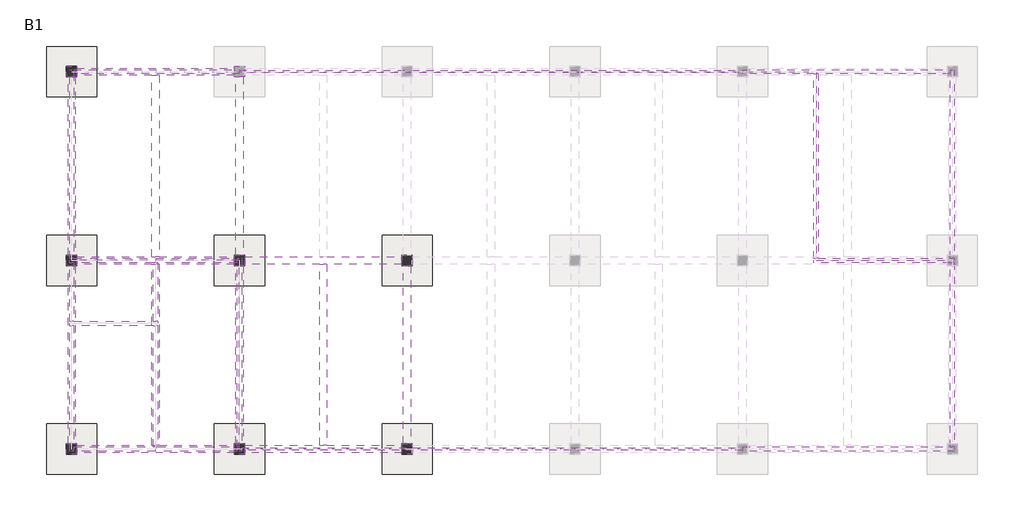
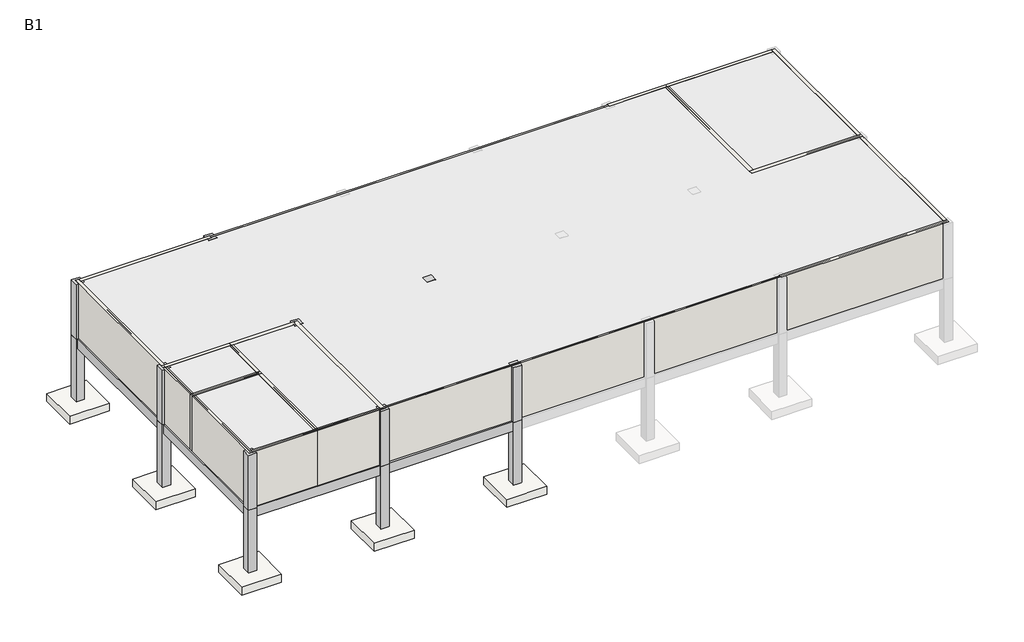
# One storey, part 1 of 2: 20 walls, 15 columns, 13 beams, 12 slabs.
# Revit data of these elements (continued)
# Elements 29, 30, 31, 32, 33 (IfcSlab, "CFS11_Slab RC_T150")
#   Height Offset From Level = 0 mm
#   Phase Created = New Construction
#   Materials on its faces: "14200-030101_Concrete Pouring"
# Elements 34, 35, 36, 37, 38, 39, 40 (IfcSlab, "FT112-Footing-Rectangular : FT112_2400x2400x500")
#   Comments = ""
#   hec_material3 = none
#   hec_material2 = none
#   hec_material1 = none
#   Structural Material = 콘크리트 - 현장타설 콘크리트
#   Phase Created = New Construction
#   Materials on its faces: "콘크리트 - 현장타설 콘크리트"
# Elements 41, 43, 46, 47, 49, 50 (IfcWall, "WA111-Exterior RC Wall 200mm")
#   Top Offset = 0 mm
#   Base Offset = 0 mm
#   Unconnected Height = 3500 mm
#   wall height = 3500 mm
#   Phase Created = New Construction
#   Base Constraint = GF
#   Materials on its faces: "Default Wall", "A03AD032-00007_Structural Concrete_25MPa-30MPa"
# Elements 42, 44, 45, 48 (IfcWall, "WA111-Exterior RC Wall 200mm")
#   Top Offset = 0 mm
#   Base Offset = 0 mm
#   Unconnected Height = 3500 mm
#   wall height = 3500 mm
#   Phase Created = New Construction
#   Base Constraint = GF
#   Materials on its faces: "A03AD032-00007_Structural Concrete_25MPa-30MPa", "Default Wall"
# Elements 51, 52 (IfcWall, "WA211_Exterior-Cement Brick-90mm")
#   Top Offset = 0 mm
#   Base Offset = 0 mm
#   Unconnected Height = 3500 mm
#   wall height = 3500 mm
#   Phase Created = New Construction
#   Base Constraint = GF
#   Materials on its faces: "Default Wall", "A04AS164-00002_Plastering_Int", "A04AS164-00001_Plastering_Ext"
# Elements 53, 56, 57, 58 (IfcWall, "WA221_Interior-Cement Block-190mm")
#   Top Offset = 0 mm
#   Base Offset = 0 mm
#   Unconnected Height = 3500 mm
#   wall height = 3500 mm
#   Phase Created = New Construction
#   Base Constraint = GF
#   Materials on its faces: "Default Wall", "A04AS164-00002_Plastering_Int"
# Elements 54, 55, 60 (IfcWall, "WA221_Interior-Cement Block-190mm")
#   Top Offset = 0 mm
#   Base Offset = 0 mm
#   Unconnected Height = 3500 mm
#   wall height = 3500 mm
#   Phase Created = New Construction
#   Base Constraint = GF
#   Materials on its faces: "A04AS164-00002_Plastering_Int", "Default Wall", "A03AD032-00007_Structural Concrete_25MPa-30MPa"
# Element 59 (IfcWall, "WA221_Interior-Cement Block-190mm")
#   Top Offset = 0 mm
#   Base Offset = 0 mm
#   Unconnected Height = 3500 mm
#   wall height = 3500 mm
#   Phase Created = New Construction
#   Base Constraint = GF
#   Materials on its faces: "Default Wall", "A04AS164-00002_Plastering_Int", "A03AD032-00007_Structural Concrete_25MPa-30MPa"
# Materials
#   "콘크리트 - 현장타설 콘크리트": class "콘크리트", colour RGB 192 192 192, transparency 0
#   "A03AE056-00001_Bitumen/Bituminous/Asphalt Coating": class "Generic", colour RGB 17 17 17, transparency 0, Description = "Damp-proofing", W00) Work Master Code = "A03AE056-00001", W01) Work Master_Lv1 = "Concrete Work", W02) Work Master_Lv2 = "Concrete Protective Coating (U/G)", W03) Work Master_Spec.1 = "Bitumen/Bituminous/Asphalt Coating", Cost = 0
#   "A03AC035-00001_Form Work (3 times in use)_Flat": class "Wood", colour RGB 149 120 74, transparency 0, Description = "Plywood", W00) Work Master Code = "A03AC035-00001", W01) Work Master_Lv1 = "Concrete Work", W02) Work Master_Lv2 = "Substructure Work", W03) Work Master_Spec.1 = "Form Work (3 times in use)", W04) Work Master_Spec.2 = "Flat Form", W05) Work Master_Spec.3 = "Dressed Lumber, Plywood or Steel Form(Wood Planks are not Allowed) incl. Chamfer", Cost = 0
#   "A03AC032-00007_Structural Concrete_Type1_25MPa-30Mpa": class "Concrete", colour RGB 176 176 176, transparency 0, Keynote = "09910.A1", Description = "Reinf. Conc.", W00) Work Master Code = "A03AC032-00007", W01) Work Master_Lv1 = "Concrete Work", W02) Work Master_Lv2 = "Substructure Work", W03) Work Master_Spec.1 = "Structural Concrete", W04) Work Master_Spec.2 = "Cement Type-1", W05) Work Master_Spec.3 = "25MPa < F'c (Cylinder Strength) ≤ 30MPa", Cost = 0
#   "14200-030101_Concrete Pouring": class "Concrete", colour RGB 176 176 176, transparency 0, Description = "Reinf. Conc.", W00) Work Master Code = "14200-030101", W01) Work Master_Lv1 = "Concrete Work", W02) Work Master_Lv2 = "Building/Shelter Foundation Work", W03) Work Master_Spec.1 = "Concrete Pouring", W04) Work Master_Spec.2 = "F'c (Cylinder Strength) > 35MPa", W05) Work Master_Spec.3 = "Cement Type-1", Cost = 0
#   "A04AL077-00001_Ext Wall Painting_Acrylic Emulsion Paint": class "Finish", colour RGB 128 128 64, transparency 0, Description = "Plastic", W00) Work Master Code = "A04AL077-00001", W01) Work Master_Lv1 = "Finishing Work", W02) Work Master_Lv2 = "Painting Work", W03) Work Master_Spec.1 = "External Wall Painting", W04) Work Master_Spec.2 = "Acrylic Emulsion Paint", Cost = 0
#   "A03AD032-00007_Structural Concrete_25MPa-30MPa": class "Concrete", colour RGB 176 176 176, transparency 0, Keynote = "09910.A1", Description = "LATEX PAINT ON F.F CONC.", W00) Work Master Code = "A03AD032-00007", W01) Work Master_Lv1 = "Concrete Work", W02) Work Master_Lv2 = "Superstructure Work", W03) Work Master_Spec.1 = "Structural Concrete", W04) Work Master_Spec.2 = "Cement Type-1", W05) Work Master_Spec.3 = "25MPa < F'c (Cylinder Strength) ≤ 30MPa", Cost = 0
#   "A03AD036-00001_Form Work (1 time in use)": class "Wood", colour RGB 149 120 74, transparency 0, Description = "Plywood", W00) Work Master Code = "A03AD036-00001", W01) Work Master_Lv1 = "Concrete Work", W02) Work Master_Lv2 = "Superstructure Work", W03) Work Master_Spec.1 = "Form Work (1 time in use)", W04) Work Master_Spec.2 = "Flat Form", W05) Work Master_Spec.3 = "Dressed Lumber, Plywood or Steel Form(Wood Planks are not Allowed) incl. Chamfer", Cost = 0
#   "A04AL078-00002_Int Wall Painting_Water Emulsion Paint": class "Finish", colour RGB 128 128 64, transparency 0, Description = "Plastic", W00) Work Master Code = "A04AL078-00002", W01) Work Master_Lv1 = "Finishing Work", W02) Work Master_Lv2 = "Painting Work", W03) Work Master_Spec.1 = "Internal Wall Painting", W04) Work Master_Spec.2 = "Water Emulsion Paint", Cost = 0
#   "A04AL081-00001_Skirt_Acrylic Emulsion Paint": class "Finish", colour RGB 128 128 64, transparency 0, Description = "Plastic", W00) Work Master Code = "A04AL081-00001", W01) Work Master_Lv1 = "Finishing Work", W02) Work Master_Lv2 = "Painting Work", W03) Work Master_Spec.1 = "Skirt Painting", W04) Work Master_Spec.2 = "Acrylic Emulsion Paint", W05) Work Master_Spec.3 = "100mm≤H<150mm", Cost = 0
#   "A04AS164-00001_Plastering_Ext": class "Concrete", colour RGB 183 186 184, transparency 0, W00) Work Master Code = "A04AS164-00001", W01) Work Master_Lv1 = "Finishing Work", W02) Work Master_Lv2 = "Plastering Work", W03) Work Master_Spec.1 = "Plastering", W04) Work Master_Spec.2 = "for External Masonry Wall", Cost = 0
#   "A04AK073-00001_Concrete Brick_0.5B": class "Concrete", colour RGB 180 180 180, transparency 0, Description = "Conc. Block", W00) Work Master Code = "A04AK073-00001", W01) Work Master_Lv1 = "Finishing Work", W02) Work Master_Lv2 = "Masonry Work", W03) Work Master_Spec.1 = "Concrete Brick", W04) Work Master_Spec.2 = "[0.5B] w/ All Reinf.(Lath, Steel Tie, Anchor Bar, Mortar, ETC.), Filler, Sealant, Lintel/Sill for Opening, ETC.", Cost = 0
#   "A04AS164-00002_Plastering_Int": class "Concrete", colour RGB 183 186 184, transparency 0, Description = "LATEX PAINT ON THK.15 CEMENT PLASTER", W00) Work Master Code = "A04AS164-00002", W01) Work Master_Lv1 = "Finishing Work", W02) Work Master_Lv2 = "Plastering Work", W03) Work Master_Spec.1 = "Plastering", W04) Work Master_Spec.2 = "for Internal Masonry Wall", Cost = 0
#   "A04AK069-00002_Reinforced Concrete Block_THK 100-200mm": class "Concrete", colour RGB 180 180 180, transparency 0, Description = "Conc. Block", W00) Work Master Code = "A04AK069-00002", W01) Work Master_Lv1 = "Finishing Work", W02) Work Master_Lv2 = "Masonry Work", W03) Work Master_Spec.1 = "Reinforced Concrete Block", W04) Work Master_Spec.2 = "w/ All Reinf.(Lath, Steel Tie, Anchor Bar, Mortar, ETC.), Filler, Sealant, Lintel/Sill for Opening, ETC.", W05) Work Master_Spec.3 = "100mm<THK≤200mm", Cost = 0
#   "Default Wall": class "Miscellaneous", colour RGB 80 80 80, transparency 0
# Room at (84209.652, 177423.861) mm, phase "New Construction", upper offset 3500 mm, lower offset 0 mm
#   Department = "EL"
#   Base Finish = ""
#   Ceiling Finish = "CL2"
#   Wall Finish = "IW2"
#   Floor Finish = "FL7"
#   Number = "0.0"
#   Name = "Battery Room"
#   Interior Finish = "IW2..N/A..N/A,,N/A..N/A,,FL7..N/A,,CL2..N/A"
#   Exterior Finish = "N/A..N/A,,EW2..N/A..N/A"
# Room at (51459.652, 168423.861) mm, phase "New Construction", upper offset 3500 mm, lower offset 0 mm
#   Department = "AR"
#   Base Finish = "WK3"
#   Ceiling Finish = ""
#   Wall Finish = "IW5"
#   Floor Finish = "FL2"
#   Number = "0.1"
#   Name = "Lobby"
#   Interior Finish = "IW5..N/A..N/A,,WK3..N/A,,FL2..N/A,,N/A..N/A"
#   Exterior Finish = "N/A..N/A,,EW2..N/A..N/A"
# Room at (66459.652, 172923.861) mm, phase "New Construction", upper offset 3500 mm, lower offset 0 mm
#   Department = "EL"
#   Base Finish = "WK1"
#   Ceiling Finish = "CL1"
#   Wall Finish = "IW5,IW2"
#   Floor Finish = "FL1"
#   Number = "0.2"
#   Name = "Cable Room"
#   Interior Finish = "IW5..IW2..N/A,,WK1..N/A,,FL1..N/A,,CL1..N/A"
#   Exterior Finish = "N/A..N/A,,EW1..EW2..N/A"
# Room at (47459.652, 166923.861) mm, phase "New Construction", upper offset 3500 mm, lower offset 0 mm
#   Department = "PATHV1"
#   Base Finish = "WK3"
#   Ceiling Finish = "CL1"
#   Wall Finish = "IW5"
#   Floor Finish = "FL2"
#   Number = "0.3"
#   Name = "Stairway"
#   Interior Finish = "IW5..N/A..N/A,,WK3..N/A,,FL2..N/A,,CL1..N/A"
#   Exterior Finish = "N/A..N/A,,EW2..N/A..N/A"
# Room at (47459.652, 171423.861) mm, phase "New Construction", upper offset 3500 mm, lower offset 0 mm
#   Department = "AR"
#   Base Finish = ""
#   Ceiling Finish = "CL3"
#   Wall Finish = ""
#   Floor Finish = ""
#   Number = "0.4"
#   Name = "Elevator"
#   Interior Finish = "N/A..N/A..N/A,,N/A..N/A,,,,CL3..N/A"
#   Exterior Finish = "N/A..N/A,,EW2..N/A..N/A"
